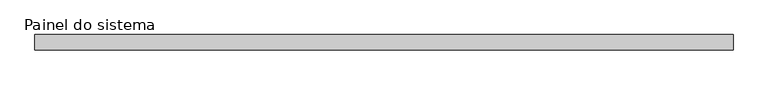
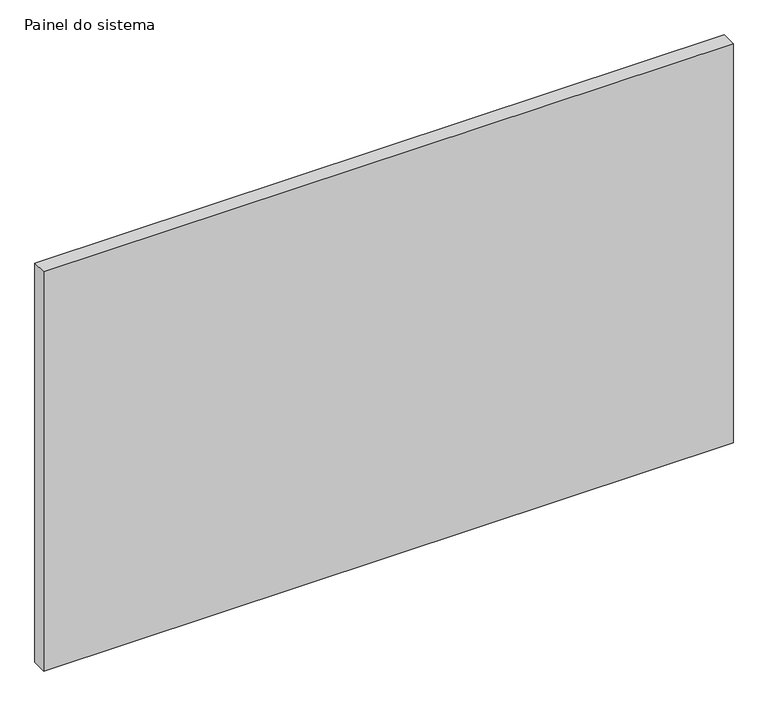
"""IFC4 building model written with IfcOpenShell, lengths in millimetres: plate geometry, Painel do sistema : Envidraçado."""

from ifc_helpers import new_model, si_unit, origin, origin_with_axes, place, context, project, spatial, polyline, outline, extrude, source, transform, mapped, element, save


def painel_do_sistema_e7d0d29a(model_context):
    return source(origin(), model_context, "Body", "SweptSolid", [
        extrude(outline(polyline([(571.8750001, -49.5), (-571.8750001, -49.5), (-571.8750001, -24.5), (571.8750001, -24.5), (571.8750001, -49.5)])), origin_with_axes(), (0.0, 0.0, 1.0), 700.0),
    ])


if __name__ == "__main__":
    model = new_model("IFC4")
    model_context = context("Model", 3, world=origin())
    ifc_project = project(units=[si_unit("LENGTHUNIT", "METRE", prefix="MILLI")], contexts=[model_context])
    site = spatial("IfcSite", under=ifc_project)
    building = spatial("IfcBuilding", under=site)
    placement = place(None, origin())
    painel_do_sistema_shape = painel_do_sistema_e7d0d29a(model_context)
    element("IfcPlate", 1, ObjectType="Painel do sistema : Envidraçado", at=placement, inside=building, context=model_context, shape_type="MappedRepresentation", body=[
        mapped(painel_do_sistema_shape, transform((0.0, 0.0, 0.0), x_axis=(1.0, 0.0, 0.0), y_axis=(0.0, 1.0, 0.0), z_axis=(0.0, 0.0, 1.0))),
    ])
    save(model, "model.ifc")

# Revit data of these elements
# Type "Painel do sistema : Envidraçado"
#   Construction Type Id = "GSP4R"
#   Analytic Construction = "Vidraça única Pilkington 1/8 pol"
#   Visual Light Transmittance = 0.9
#   Solar Heat Gain Coefficient = 0.86
#   Heat Transfer Coefficient (U) = 6.7069 W/(m²·K)
# Element 1 (IfcPlate, "Painel do sistema : Envidraçado")
#   Materials on its faces: ".VIDRO GENÉRICO"
# Materials
#   ".VIDRO GENÉRICO": class ".CC_VIDRO", colour RGB 0 128 192, transparency 0.9, Description = "Vidro comum", Cost = 0
